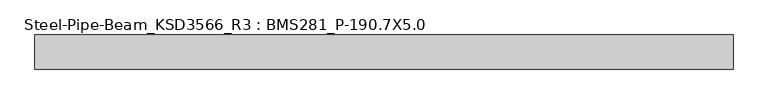
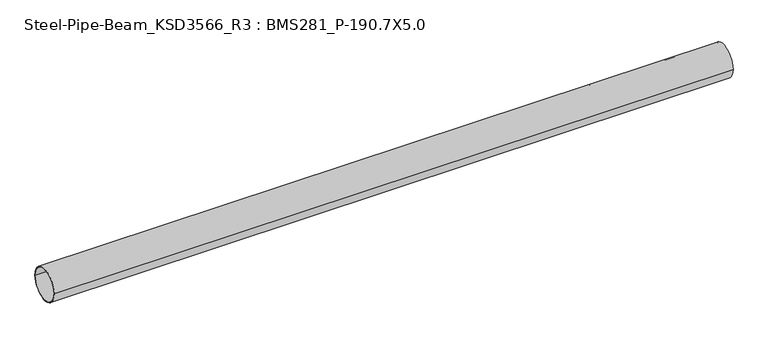
"""IFC4 building model written with IfcOpenShell, lengths in millimetres: member geometry, Steel-Pipe-Beam_KSD3566_R3 : BMS281_P-190.7X5.0."""

import ifcopenshell
import ifcopenshell.guid

model = None  # the IFC model being written
_history = None  # IfcOwnerHistory: only IFC2X3 demands one
_inside = {}  # id of a spatial element -> (the spatial element, [elements in it])
_under = {}  # id of a project, library or spatial element -> (it, [spatial elements below it])
_declared = {}  # id of a project -> (the project, [libraries it declares])
_typed = {}  # id of a type object -> (the type object, [elements of that type])
_made_of = {}  # id of a material, layer set ... -> (it, [elements and type objects made of it])


def new_model(schema):
    """Start an empty IFC model of exactly this schema.

    Asked for "IFC4X3", IfcOpenShell would pick the latest addendum, in which some entities
    have other attributes; the version numbers below select the first issue.
    IFC2X3 requires an IfcOwnerHistory on every rooted entity: one is made here for all.
    """
    global model, _history
    if schema == "IFC4X3":
        model = ifcopenshell.file(schema_version=(4, 3, 0, 0))
    else:
        model = ifcopenshell.file(schema=schema)
    _inside.clear()
    _under.clear()
    _declared.clear()
    _typed.clear()
    _made_of.clear()
    _history = None
    if model.schema == "IFC2X3":
        org = make("IfcOrganization", Name="unknown")
        user = make(
            "IfcPersonAndOrganization",
            ThePerson=make("IfcPerson", FamilyName="unknown"),
            TheOrganization=org,
        )
        app = make(
            "IfcApplication",
            ApplicationDeveloper=org,
            Version="unknown",
            ApplicationFullName="unknown",
            ApplicationIdentifier="unknown",
        )
        _history = make(
            "IfcOwnerHistory",
            OwningUser=user,
            OwningApplication=app,
            ChangeAction="ADDED",
            CreationDate=0,
        )
    return model


def make(cls, **values):
    """One entity of the class cls with the attributes given. An attribute that is None is left unset."""
    return model.create_entity(
        cls, **{name: value for name, value in values.items() if value is not None}
    )


def rooted(cls, **values):
    """An entity with a GlobalId (a new one), such as an element, a storey or a relation."""
    return make(cls, GlobalId=ifcopenshell.guid.new(), OwnerHistory=_history, **values)


def si_unit(unit_type, name, prefix=None):
    """IfcSIUnit, for example si_unit("LENGTHUNIT", "METRE", prefix="MILLI")."""
    return make("IfcSIUnit", UnitType=unit_type, Prefix=prefix, Name=name)


def assignment(units):
    """IfcUnitAssignment: the units of a project."""
    return None if units is None else make("IfcUnitAssignment", Units=units)


def point(xyz):
    """IfcCartesianPoint."""
    return None if xyz is None else make("IfcCartesianPoint", Coordinates=xyz)


def direction(xyz):
    """IfcDirection."""
    return None if xyz is None else make("IfcDirection", DirectionRatios=xyz)


def frame(location, z_axis=None, x_axis=None):
    """IfcAxis2Placement3D, a coordinate frame: its origin and axes. An axis left out is left unset."""
    return make(
        "IfcAxis2Placement3D",
        Location=point(location),
        Axis=direction(z_axis),
        RefDirection=direction(x_axis),
    )


def frame_2d(location, x_axis=None):
    """IfcAxis2Placement2D, a coordinate frame in the plane: its origin and x axis."""
    return make(
        "IfcAxis2Placement2D", Location=point(location), RefDirection=direction(x_axis)
    )


def origin():
    """The frame at (0, 0, 0) with its axes left unset."""
    return frame((0.0, 0.0, 0.0))


def origin_2d():
    """The frame at (0, 0) in the plane with its x axis left unset."""
    return frame_2d((0.0, 0.0))


def place(relative_to, where):
    """IfcLocalPlacement: puts the frame where relative to a parent placement (None: the world)."""
    return make(
        "IfcLocalPlacement", PlacementRelTo=relative_to, RelativePlacement=where
    )


def context(
    kind, dimensions, precision=None, world=None, true_north=None, identifier=None
):
    """IfcGeometricRepresentationContext, for example the 3D "Model" context."""
    return make(
        "IfcGeometricRepresentationContext",
        ContextIdentifier=identifier,
        ContextType=kind,
        CoordinateSpaceDimension=dimensions,
        Precision=precision,
        WorldCoordinateSystem=world,
        TrueNorth=true_north,
    )


def project(units=None, contexts=None):
    """IfcProject with its units and contexts."""
    return rooted(
        "IfcProject",
        Name="project",
        RepresentationContexts=contexts,
        UnitsInContext=assignment(units),
    )


def spatial(cls, under=None, at=None, **own):
    """A site, building, storey or space (cls), placed at a placement, below another one or the project."""
    s = rooted(cls, ObjectPlacement=at, **own)
    if under is not None:
        _under.setdefault(under.id(), (under, []))[1].append(s)
    return s


def circle_curve(where, radius):
    """IfcCircle in the frame where."""
    return make("IfcCircle", Position=where, Radius=radius)


def trimmed(basis, trim1, trim2, sense, master):
    """IfcTrimmedCurve: the piece of a basis curve between two trims."""
    return make(
        "IfcTrimmedCurve",
        BasisCurve=basis,
        Trim1=trim1,
        Trim2=trim2,
        SenseAgreement=sense,
        MasterRepresentation=master,
    )


def segment(curve, same_sense, transition):
    """IfcCompositeCurveSegment."""
    return make(
        "IfcCompositeCurveSegment",
        Transition=transition,
        SameSense=same_sense,
        ParentCurve=curve,
    )


def composite_curve(segments, self_intersect=None):
    """IfcCompositeCurve: segments joined end to end."""
    return make("IfcCompositeCurve", Segments=segments, SelfIntersect=self_intersect)


def outline(outer, holes=None, kind="AREA"):
    """IfcArbitraryClosedProfileDef: a profile drawn as a closed curve; with holes, ...WithVoids."""
    if holes is None:
        return make("IfcArbitraryClosedProfileDef", ProfileType=kind, OuterCurve=outer)
    return make(
        "IfcArbitraryProfileDefWithVoids",
        ProfileType=kind,
        OuterCurve=outer,
        InnerCurves=holes,
    )


def extrude(swept, where, along, depth):
    """IfcExtrudedAreaSolid: the profile swept, set in the frame where, extruded along a direction by depth."""
    return make(
        "IfcExtrudedAreaSolid",
        SweptArea=swept,
        Position=where,
        ExtrudedDirection=direction(along),
        Depth=depth,
    )


def shape(context_of_items, identifier, shape_type, items):
    """IfcShapeRepresentation: the items that make up one representation, for example the "Body"."""
    return make(
        "IfcShapeRepresentation",
        ContextOfItems=context_of_items,
        RepresentationIdentifier=identifier,
        RepresentationType=shape_type,
        Items=items,
    )


def source(mapping_origin, context_of_items, identifier, shape_type, items):
    """IfcRepresentationMap: a shape defined once, which mapped items show again and again."""
    return make(
        "IfcRepresentationMap",
        MappingOrigin=mapping_origin,
        MappedRepresentation=shape(context_of_items, identifier, shape_type, items),
    )


def transform(
    local_origin,
    x_axis=None,
    y_axis=None,
    z_axis=None,
    scale=None,
    scale2=None,
    scale3=None,
    uniform=True,
):
    """IfcCartesianTransformationOperator3D, or its non-uniform kind. x_axis, y_axis, z_axis: its Axis1, 2, 3."""
    if uniform:
        return make(
            "IfcCartesianTransformationOperator3D",
            Axis1=direction(x_axis),
            Axis2=direction(y_axis),
            LocalOrigin=point(local_origin),
            Scale=scale,
            Axis3=direction(z_axis),
        )
    return make(
        "IfcCartesianTransformationOperator3DnonUniform",
        Axis1=direction(x_axis),
        Axis2=direction(y_axis),
        LocalOrigin=point(local_origin),
        Scale=scale,
        Axis3=direction(z_axis),
        Scale2=scale2,
        Scale3=scale3,
    )


def mapped(mapping_source, mapping_target):
    """IfcMappedItem: shows the shape of a source again, moved by a transform."""
    return make(
        "IfcMappedItem", MappingSource=mapping_source, MappingTarget=mapping_target
    )


def made_of(thing, what):
    """Note that an element or type object is made of a material, layer set ...; save() writes the relation."""
    if what is not None:
        _made_of.setdefault(what.id(), (what, []))[1].append(thing)
    return thing


def element(
    cls,
    number,
    at=None,
    inside=None,
    cuts=None,
    type_object=None,
    material=None,
    context=None,
    identifier="Body",
    shape_type=None,
    held_by="IfcProductDefinitionShape",
    body=None,
    shapes=None,
    **own,
):
    """One element of the class cls, such as IfcWall. Its Tag is "e" and its number.

    at: its placement. inside: the storey or other place that contains it. cuts: it is an
    opening in that element (IfcRelVoidsElement). A single representation is given by context,
    identifier, shape_type and body (its items); several are given by shapes. held_by: the class
    of the entity that holds the representations. save() writes the other relations.
    """
    e = rooted(cls, Tag="e%d" % number, ObjectPlacement=at, **own)
    if body is not None:
        shapes = [shape(context, identifier, shape_type, body)]
    if shapes is not None:
        e.Representation = make(held_by, Representations=shapes)
    if inside is not None:
        _inside.setdefault(inside.id(), (inside, []))[1].append(e)
    if cuts is not None:
        rooted(
            "IfcRelVoidsElement", RelatingBuildingElement=cuts, RelatedOpeningElement=e
        )
    if type_object is not None:
        _typed.setdefault(type_object.id(), (type_object, []))[1].append(e)
    return made_of(e, material)


def aggregate(whole, parts):
    """IfcRelAggregates: a whole, such as a stair, and the parts it consists of."""
    return rooted("IfcRelAggregates", RelatingObject=whole, RelatedObjects=parts)


def save(model, path):
    """Write the relations noted so far, then the file.

    IfcRelAggregates (storeys below a building ...), IfcRelContainedInSpatialStructure (elements
    in a storey), IfcRelDefinesByType, IfcRelAssociatesMaterial and IfcRelDeclares: one each for
    every whole, place, type object, material and project.
    """
    for whole, parts in _under.values():
        aggregate(whole, parts)
    for where, things in _inside.values():
        rooted(
            "IfcRelContainedInSpatialStructure",
            RelatedElements=things,
            RelatingStructure=where,
        )
    for kind, things in _typed.values():
        rooted("IfcRelDefinesByType", RelatedObjects=things, RelatingType=kind)
    for what, things in _made_of.values():
        rooted("IfcRelAssociatesMaterial", RelatedObjects=things, RelatingMaterial=what)
    for by, libraries in _declared.values():
        rooted("IfcRelDeclares", RelatingContext=by, RelatedDefinitions=libraries)
    model.write(path)


def steel_pipe_beam_ksd3566_r3_bms281_p_190_7x5_0_634dc5dd(model_context):
    return source(origin(), model_context, "Body", "SweptSolid", [
        extrude(outline(composite_curve([segment(trimmed(circle_curve(origin_2d(), 95.35), [point((-95.35, 0.0))], [point((95.35, 0.0))], False, "CARTESIAN"), True, "CONTINUOUS"), segment(trimmed(circle_curve(origin_2d(), 95.35), [point((95.35, 0.0))], [point((-95.35, 0.0))], False, "CARTESIAN"), True, "CONTINUOUS")], self_intersect=False), holes=[composite_curve([segment(trimmed(circle_curve(origin_2d(), 90.35), [point((90.35, 0.0))], [point((-90.35, 0.0))], True, "CARTESIAN"), True, "CONTINUOUS"), segment(trimmed(circle_curve(origin_2d(), 90.35), [point((-90.35, 0.0))], [point((90.35, 0.0))], True, "CARTESIAN"), True, "CONTINUOUS")], self_intersect=False)]), frame((-1932.8589545, 0.0, 0.0), z_axis=(1.0, 0.0, 0.0), x_axis=(0.0, 1.0, 0.0)), (0.0, 0.0, 1.0), 3898.3272248),
    ])


if __name__ == "__main__":
    model = new_model("IFC4")
    model_context = context("Model", 3, world=origin())
    ifc_project = project(units=[si_unit("LENGTHUNIT", "METRE", prefix="MILLI")], contexts=[model_context])
    site = spatial("IfcSite", under=ifc_project)
    building = spatial("IfcBuilding", under=site)
    placement = place(None, origin())
    steel_pipe_beam_ksd3566_r3_bms281_p_190_7x5_0_shape = steel_pipe_beam_ksd3566_r3_bms281_p_190_7x5_0_634dc5dd(model_context)
    element("IfcMember", 1, ObjectType="Steel-Pipe-Beam_KSD3566_R3 : BMS281_P-190.7X5.0", at=placement, inside=building, context=model_context, shape_type="MappedRepresentation", body=[
        mapped(steel_pipe_beam_ksd3566_r3_bms281_p_190_7x5_0_shape, transform((0.0, 0.0, 0.0), x_axis=(1.0, 0.0, 0.0), y_axis=(0.0, 1.0, 0.0), z_axis=(0.0, 0.0, 1.0))),
    ])
    save(model, "model.ifc")

# Revit data of these elements
# Type "Steel-Pipe-Beam_KSD3566_R3 : BMS281_P-190.7X5.0"
#   Keynote = "P-190.7X5.0"
#   SteelWeight = "Light"
#   t = 0.0050 m
#   Surface Area = 0.599102 m²/m
#   Section Area = 29.1697 cm²
#   Mass per Unit Length = 22.8982 kg/m
#   Length [instance default] = 1.5000 m
#   D = 0.1907 m
#   hec_material4 [instance default] = none
#   hec_material3 [instance default] = none
#   hec_material2 [instance default] = none
#   hec_material1 [instance default] = none
#   Structural Material [instance default] = Steel, 45-345
#   Assembly Code = ""
# Element 1 (IfcMember, "Steel-Pipe-Beam_KSD3566_R3 : BMS281_P-190.7X5.0")
#   Structural Material = none
# Materials
#   "Steel, 45-345": class "Metal", colour RGB 189 187 185, transparency 0, Description = "Steel 345 MPa", Cost = 0
